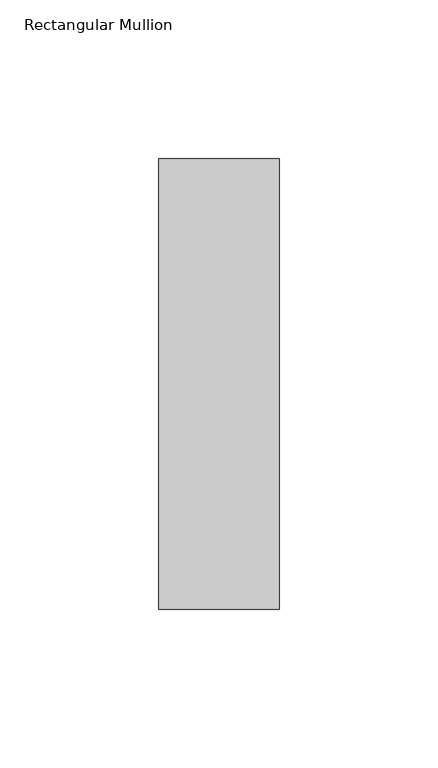
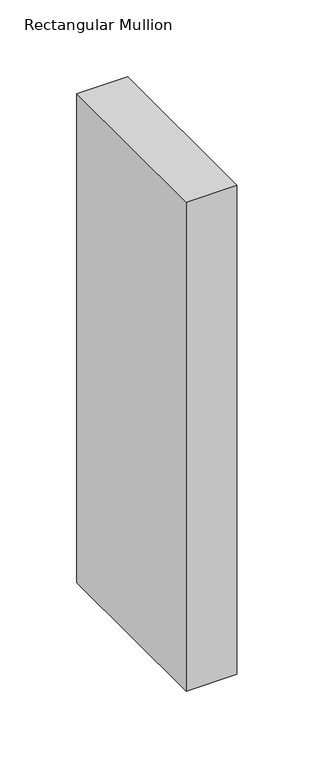
"""IFC4 building model written with IfcOpenShell, lengths in millimetres: member geometry, Rectangular Mullion : NLRS_21_CWM_hsb-regel 38x142_gen_rsf."""

from ifc_helpers import new_model, si_unit, frame, origin, place, context, project, spatial, polyline, outline, extrude, source, transform, mapped, element, save


def rectangular_mullion_05042751(model_context):
    return source(origin(), model_context, "Body", "SweptSolid", [
        extrude(outline(polyline([(19.0, -71.0), (-19.0, -71.0), (-19.0, 71.0), (19.0, 71.0), (19.0, -71.0)])), frame((0.0, 0.0, -388.0), z_axis=(0.0, 0.0, 1.0), x_axis=(1.0, 0.0, 0.0)), (0.0, 0.0, 1.0), 388.0),
    ])


if __name__ == "__main__":
    model = new_model("IFC4")
    model_context = context("Model", 3, world=origin())
    ifc_project = project(units=[si_unit("LENGTHUNIT", "METRE", prefix="MILLI")], contexts=[model_context])
    site = spatial("IfcSite", under=ifc_project)
    building = spatial("IfcBuilding", under=site)
    placement = place(None, origin())
    rectangular_mullion_shape = rectangular_mullion_05042751(model_context)
    element("IfcMember", 1, ObjectType="Rectangular Mullion : NLRS_21_CWM_hsb-regel 38x142_gen_rsf", at=placement, inside=building, context=model_context, shape_type="MappedRepresentation", body=[
        mapped(rectangular_mullion_shape, transform((0.0, 0.0, 0.0), x_axis=(1.0, 0.0, 0.0), y_axis=(0.0, 1.0, 0.0), z_axis=(0.0, 0.0, 1.0))),
    ])
    save(model, "model.ifc")

# Revit data of these elements
# Type "Rectangular Mullion : NLRS_21_CWM_hsb-regel 38x142_gen_rsf"
#   Export Type to IFC As = "IfcWall"
#   Type IfcGUID = "07M7mRoiH1CR8m_RSKIwpF"
#   Assembly Code = "21.10"
#   built-in parameter 1007322 = 0.465879 (stored number, unit not read)
#   built-in parameter 1007321 = 0.062336 (stored number, unit not read)
#   built-in parameter 1007320 = 0.062336 (stored number, unit not read)
# Element 1 (IfcMember, "Rectangular Mullion : NLRS_21_CWM_hsb-regel 38x142_gen_rsf")
#   Materials on its faces: "NLRS_i2_hout naaldhout vuren_gen_rsf"
# Materials
#   "NLRS_i2_hout naaldhout vuren_gen_rsf": class "I - Hout", colour RGB 234 199 147, transparency 0, Keynote = "i2", Manufacturer = "Revit Standards Foundation", URL = "www.revitstandards.org", Description = "hout vuren", Cost = 0
